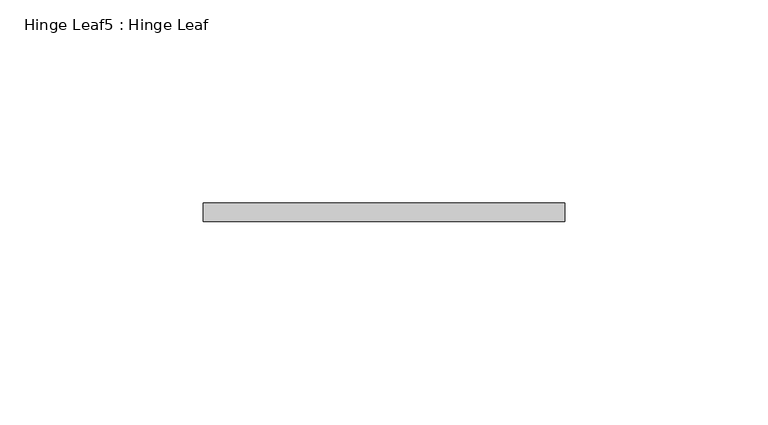
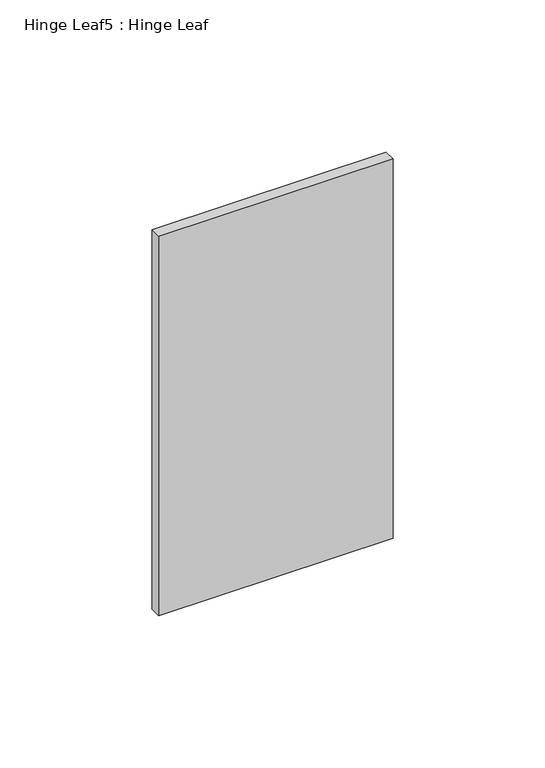
"""IFC4 building model written with IfcOpenShell, lengths in millimetres: proxy geometry, Hinge Leaf5 : Hinge Leaf."""

from ifc_helpers import new_model, si_unit, frame, origin, place, context, project, spatial, polyline, outline, extrude, source, transform, mapped, element, save


def hinge_leaf5_hinge_leaf_6d526917(model_context):
    return source(origin(), model_context, "Body", "SweptSolid", [
        extrude(outline(polyline([(587327.7934739, -531772.5663841), (587416.6934739, -531772.5663841), (587416.6934739, -531777.1383841), (587327.7934739, -531777.1383841), (587327.7934739, -531772.5663841)])), frame((0.0, 0.0, 1936.75), z_axis=(0.0, 0.0, 1.0), x_axis=(1.0, 0.0, 0.0)), (0.0, 0.0, 1.0), 152.4),
    ])


if __name__ == "__main__":
    model = new_model("IFC4")
    model_context = context("Model", 3, world=origin())
    ifc_project = project(units=[si_unit("LENGTHUNIT", "METRE", prefix="MILLI")], contexts=[model_context])
    site = spatial("IfcSite", under=ifc_project)
    building = spatial("IfcBuilding", under=site)
    placement = place(None, origin())
    hinge_leaf5_hinge_leaf_shape = hinge_leaf5_hinge_leaf_6d526917(model_context)
    element("IfcBuildingElementProxy", 1, Name="Hinge Leaf5 : Hinge Leaf", ObjectType="Hinge Leaf5 : Hinge Leaf", at=placement, inside=building, context=model_context, shape_type="MappedRepresentation", body=[
        mapped(hinge_leaf5_hinge_leaf_shape, transform((0.0, 0.0, 0.0), x_axis=(1.0, 0.0, 0.0), y_axis=(0.0, 1.0, 0.0), z_axis=(0.0, 0.0, 1.0))),
    ])
    save(model, "model.ifc")

# Revit data of these elements
# Element 1 (IfcBuildingElementProxy, "Hinge Leaf5 : Hinge Leaf")
#   Materials on its faces: "6\"X6\" WELD-ON STL BUTT HINGE"
# Materials
#   "6\"X6\" WELD-ON STL BUTT HINGE": class "Metal", colour RGB 189 187 185, transparency 0, Description = "Carbon steel", Cost = 0
